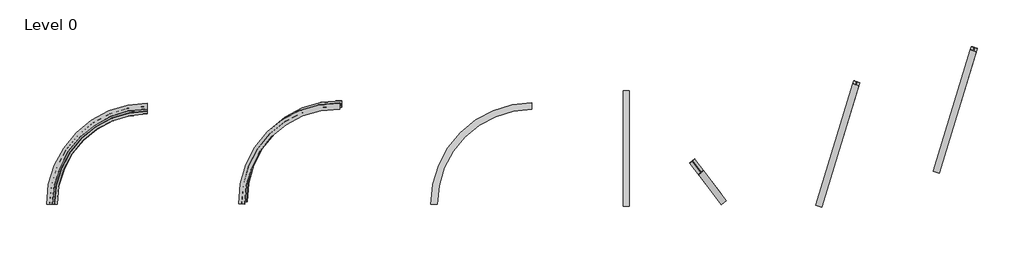
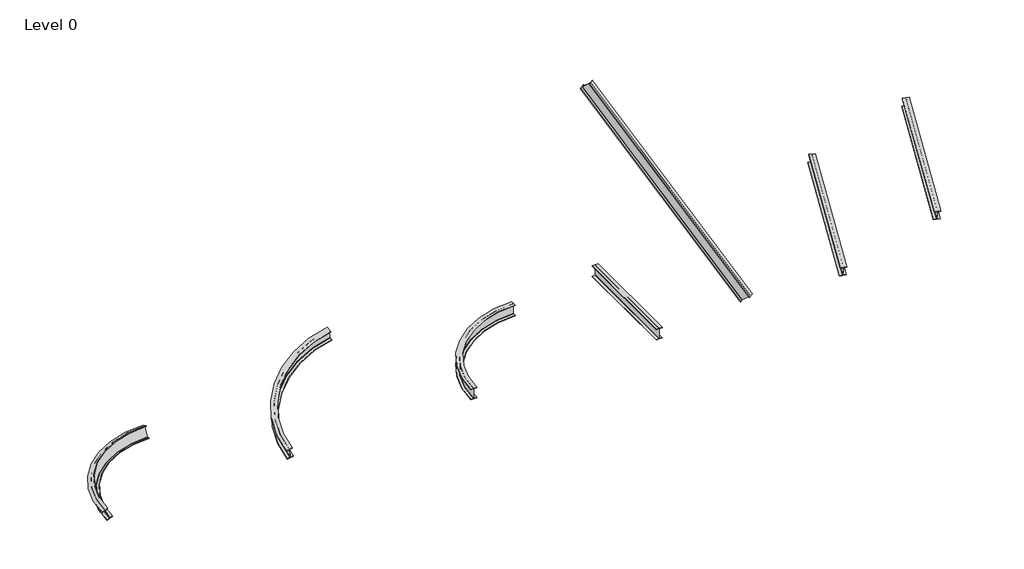
# One storey: 7 beams.
"""IFC4 building model written with IfcOpenShell, lengths in millimetres."""

import ifcopenshell
import ifcopenshell.guid

model = None  # the IFC model being written
_history = None  # IfcOwnerHistory: only IFC2X3 demands one
_inside = {}  # id of a spatial element -> (the spatial element, [elements in it])
_under = {}  # id of a project, library or spatial element -> (it, [spatial elements below it])
_declared = {}  # id of a project -> (the project, [libraries it declares])
_typed = {}  # id of a type object -> (the type object, [elements of that type])
_made_of = {}  # id of a material, layer set ... -> (it, [elements and type objects made of it])


def new_model(schema):
    """Start an empty IFC model of exactly this schema.

    Asked for "IFC4X3", IfcOpenShell would pick the latest addendum, in which some entities
    have other attributes; the version numbers below select the first issue.
    IFC2X3 requires an IfcOwnerHistory on every rooted entity: one is made here for all.
    """
    global model, _history
    if schema == "IFC4X3":
        model = ifcopenshell.file(schema_version=(4, 3, 0, 0))
    else:
        model = ifcopenshell.file(schema=schema)
    _inside.clear()
    _under.clear()
    _declared.clear()
    _typed.clear()
    _made_of.clear()
    _history = None
    if model.schema == "IFC2X3":
        org = make("IfcOrganization", Name="unknown")
        user = make(
            "IfcPersonAndOrganization",
            ThePerson=make("IfcPerson", FamilyName="unknown"),
            TheOrganization=org,
        )
        app = make(
            "IfcApplication",
            ApplicationDeveloper=org,
            Version="unknown",
            ApplicationFullName="unknown",
            ApplicationIdentifier="unknown",
        )
        _history = make(
            "IfcOwnerHistory",
            OwningUser=user,
            OwningApplication=app,
            ChangeAction="ADDED",
            CreationDate=0,
        )
    return model


def make(cls, **values):
    """One entity of the class cls with the attributes given. An attribute that is None is left unset."""
    return model.create_entity(
        cls, **{name: value for name, value in values.items() if value is not None}
    )


def rooted(cls, **values):
    """An entity with a GlobalId (a new one), such as an element, a storey or a relation."""
    return make(cls, GlobalId=ifcopenshell.guid.new(), OwnerHistory=_history, **values)


def si_unit(unit_type, name, prefix=None):
    """IfcSIUnit, for example si_unit("LENGTHUNIT", "METRE", prefix="MILLI")."""
    return make("IfcSIUnit", UnitType=unit_type, Prefix=prefix, Name=name)


def assignment(units):
    """IfcUnitAssignment: the units of a project."""
    return None if units is None else make("IfcUnitAssignment", Units=units)


def point(xyz):
    """IfcCartesianPoint."""
    return None if xyz is None else make("IfcCartesianPoint", Coordinates=xyz)


def direction(xyz):
    """IfcDirection."""
    return None if xyz is None else make("IfcDirection", DirectionRatios=xyz)


def frame(location, z_axis=None, x_axis=None):
    """IfcAxis2Placement3D, a coordinate frame: its origin and axes. An axis left out is left unset."""
    return make(
        "IfcAxis2Placement3D",
        Location=point(location),
        Axis=direction(z_axis),
        RefDirection=direction(x_axis),
    )


def frame_2d(location, x_axis=None):
    """IfcAxis2Placement2D, a coordinate frame in the plane: its origin and x axis."""
    return make(
        "IfcAxis2Placement2D", Location=point(location), RefDirection=direction(x_axis)
    )


def origin():
    """The frame at (0, 0, 0) with its axes left unset."""
    return frame((0.0, 0.0, 0.0))


def place(relative_to, where):
    """IfcLocalPlacement: puts the frame where relative to a parent placement (None: the world)."""
    return make(
        "IfcLocalPlacement", PlacementRelTo=relative_to, RelativePlacement=where
    )


def context(
    kind, dimensions, precision=None, world=None, true_north=None, identifier=None
):
    """IfcGeometricRepresentationContext, for example the 3D "Model" context."""
    return make(
        "IfcGeometricRepresentationContext",
        ContextIdentifier=identifier,
        ContextType=kind,
        CoordinateSpaceDimension=dimensions,
        Precision=precision,
        WorldCoordinateSystem=world,
        TrueNorth=true_north,
    )


def project(units=None, contexts=None):
    """IfcProject with its units and contexts."""
    return rooted(
        "IfcProject",
        Name="project",
        RepresentationContexts=contexts,
        UnitsInContext=assignment(units),
    )


def spatial(cls, under=None, at=None, **own):
    """A site, building, storey or space (cls), placed at a placement, below another one or the project."""
    s = rooted(cls, ObjectPlacement=at, **own)
    if under is not None:
        _under.setdefault(under.id(), (under, []))[1].append(s)
    return s


def polyline(points):
    """IfcPolyline through the points."""
    return make("IfcPolyline", Points=[point(p) for p in points])


def circle_curve(where, radius):
    """IfcCircle in the frame where."""
    return make("IfcCircle", Position=where, Radius=radius)


def ellipse_curve(where, semi_axis1, semi_axis2):
    """IfcEllipse in the frame where."""
    return make(
        "IfcEllipse", Position=where, SemiAxis1=semi_axis1, SemiAxis2=semi_axis2
    )


def trimmed(basis, trim1, trim2, sense, master):
    """IfcTrimmedCurve: the piece of a basis curve between two trims."""
    return make(
        "IfcTrimmedCurve",
        BasisCurve=basis,
        Trim1=trim1,
        Trim2=trim2,
        SenseAgreement=sense,
        MasterRepresentation=master,
    )


def segment(curve, same_sense, transition):
    """IfcCompositeCurveSegment."""
    return make(
        "IfcCompositeCurveSegment",
        Transition=transition,
        SameSense=same_sense,
        ParentCurve=curve,
    )


def composite_curve(segments, self_intersect=None):
    """IfcCompositeCurve: segments joined end to end."""
    return make("IfcCompositeCurve", Segments=segments, SelfIntersect=self_intersect)


def outline(outer, holes=None, kind="AREA"):
    """IfcArbitraryClosedProfileDef: a profile drawn as a closed curve; with holes, ...WithVoids."""
    if holes is None:
        return make("IfcArbitraryClosedProfileDef", ProfileType=kind, OuterCurve=outer)
    return make(
        "IfcArbitraryProfileDefWithVoids",
        ProfileType=kind,
        OuterCurve=outer,
        InnerCurves=holes,
    )


def extrude(swept, where, along, depth):
    """IfcExtrudedAreaSolid: the profile swept, set in the frame where, extruded along a direction by depth."""
    return make(
        "IfcExtrudedAreaSolid",
        SweptArea=swept,
        Position=where,
        ExtrudedDirection=direction(along),
        Depth=depth,
    )


def shape(context_of_items, identifier, shape_type, items):
    """IfcShapeRepresentation: the items that make up one representation, for example the "Body"."""
    return make(
        "IfcShapeRepresentation",
        ContextOfItems=context_of_items,
        RepresentationIdentifier=identifier,
        RepresentationType=shape_type,
        Items=items,
    )


def source(mapping_origin, context_of_items, identifier, shape_type, items):
    """IfcRepresentationMap: a shape defined once, which mapped items show again and again."""
    return make(
        "IfcRepresentationMap",
        MappingOrigin=mapping_origin,
        MappedRepresentation=shape(context_of_items, identifier, shape_type, items),
    )


def transform(
    local_origin,
    x_axis=None,
    y_axis=None,
    z_axis=None,
    scale=None,
    scale2=None,
    scale3=None,
    uniform=True,
):
    """IfcCartesianTransformationOperator3D, or its non-uniform kind. x_axis, y_axis, z_axis: its Axis1, 2, 3."""
    if uniform:
        return make(
            "IfcCartesianTransformationOperator3D",
            Axis1=direction(x_axis),
            Axis2=direction(y_axis),
            LocalOrigin=point(local_origin),
            Scale=scale,
            Axis3=direction(z_axis),
        )
    return make(
        "IfcCartesianTransformationOperator3DnonUniform",
        Axis1=direction(x_axis),
        Axis2=direction(y_axis),
        LocalOrigin=point(local_origin),
        Scale=scale,
        Axis3=direction(z_axis),
        Scale2=scale2,
        Scale3=scale3,
    )


def mapped(mapping_source, mapping_target):
    """IfcMappedItem: shows the shape of a source again, moved by a transform."""
    return make(
        "IfcMappedItem", MappingSource=mapping_source, MappingTarget=mapping_target
    )


def made_of(thing, what):
    """Note that an element or type object is made of a material, layer set ...; save() writes the relation."""
    if what is not None:
        _made_of.setdefault(what.id(), (what, []))[1].append(thing)
    return thing


def element(
    cls,
    number,
    at=None,
    inside=None,
    cuts=None,
    type_object=None,
    material=None,
    context=None,
    identifier="Body",
    shape_type=None,
    held_by="IfcProductDefinitionShape",
    body=None,
    shapes=None,
    **own,
):
    """One element of the class cls, such as IfcWall. Its Tag is "e" and its number.

    at: its placement. inside: the storey or other place that contains it. cuts: it is an
    opening in that element (IfcRelVoidsElement). A single representation is given by context,
    identifier, shape_type and body (its items); several are given by shapes. held_by: the class
    of the entity that holds the representations. save() writes the other relations.
    """
    e = rooted(cls, Tag="e%d" % number, ObjectPlacement=at, **own)
    if body is not None:
        shapes = [shape(context, identifier, shape_type, body)]
    if shapes is not None:
        e.Representation = make(held_by, Representations=shapes)
    if inside is not None:
        _inside.setdefault(inside.id(), (inside, []))[1].append(e)
    if cuts is not None:
        rooted(
            "IfcRelVoidsElement", RelatingBuildingElement=cuts, RelatedOpeningElement=e
        )
    if type_object is not None:
        _typed.setdefault(type_object.id(), (type_object, []))[1].append(e)
    return made_of(e, material)


def aggregate(whole, parts):
    """IfcRelAggregates: a whole, such as a stair, and the parts it consists of."""
    return rooted("IfcRelAggregates", RelatingObject=whole, RelatedObjects=parts)


def save(model, path):
    """Write the relations noted so far, then the file.

    IfcRelAggregates (storeys below a building ...), IfcRelContainedInSpatialStructure (elements
    in a storey), IfcRelDefinesByType, IfcRelAssociatesMaterial and IfcRelDeclares: one each for
    every whole, place, type object, material and project.
    """
    for whole, parts in _under.values():
        aggregate(whole, parts)
    for where, things in _inside.values():
        rooted(
            "IfcRelContainedInSpatialStructure",
            RelatedElements=things,
            RelatingStructure=where,
        )
    for kind, things in _typed.values():
        rooted("IfcRelDefinesByType", RelatedObjects=things, RelatingType=kind)
    for what, things in _made_of.values():
        rooted("IfcRelAssociatesMaterial", RelatedObjects=things, RelatingMaterial=what)
    for by, libraries in _declared.values():
        rooted("IfcRelDeclares", RelatingContext=by, RelatedDefinitions=libraries)
    model.write(path)


def plane_surface(at):
    """IfcPlane: the flat surface through the origin of the frame at, square to its z axis."""
    return make("IfcPlane", Position=at)


def cylinder_surface(at, radius):
    """IfcCylindricalSurface: all points at the distance radius from the z axis of the frame at."""
    return make("IfcCylindricalSurface", Position=at, Radius=radius)


def revolved_surface(curve, axis_point, axis_direction):
    """IfcSurfaceOfRevolution: the curve turned about the line through axis_point along axis_direction."""
    return make(
        "IfcSurfaceOfRevolution",
        SweptCurve=make("IfcArbitraryOpenProfileDef", ProfileType="CURVE", Curve=curve),
        AxisPosition=make("IfcAxis1Placement", Location=point(axis_point), Axis=direction(axis_direction)),
    )


def advanced_brep(points, edges, surfaces, faces):
    """IfcAdvancedBrep: a solid bounded by faces that lie on surfaces and meet in shared edges.

    An edge is (start, end): straight between two places in points (the first is 0);
    or (start, end, curve); or (start, end, curve, False) where it runs against its curve.
    A face is (place in surfaces, loops), or (place, loops, False) where it looks against
    its surface's normal. A loop lists edges by number (the first is 1), with a minus sign
    where the edge is run from its end to its start. The first loop is the outer one.
    """
    corners = [point(p) for p in points]
    vertices = [make("IfcVertexPoint", VertexGeometry=c) for c in corners]
    made = []
    for start, end, *more in edges:
        made.append(
            make(
                "IfcEdgeCurve",
                EdgeStart=vertices[start],
                EdgeEnd=vertices[end],
                EdgeGeometry=more[0] if more else make("IfcPolyline", Points=[corners[start], corners[end]]),
                SameSense=more[1] if len(more) > 1 else True,
            )
        )
    hull = []
    for where, loops, *sense in faces:
        bounds = []
        for j, loop in enumerate(loops):
            ring = [make("IfcOrientedEdge", EdgeElement=made[abs(k) - 1], Orientation=k > 0) for k in loop]
            bounds.append(
                make(
                    "IfcFaceOuterBound" if j == 0 else "IfcFaceBound",
                    Bound=make("IfcEdgeLoop", EdgeList=ring),
                    Orientation=True,
                )
            )
        hull.append(make("IfcAdvancedFace", Bounds=bounds, FaceSurface=surfaces[where], SameSense=sense[0] if sense else True))
    return make("IfcAdvancedBrep", Outer=make("IfcClosedShell", CfsFaces=hull))


def ub_universal_beams_ub305x165x40_8b2c45c1(model_context):
    return source(origin(), model_context, "Body", "SweptSolid", [
        extrude(outline(composite_curve([segment(polyline([(82.5, -141.5), (82.5, -151.7), (-82.5, -151.7), (-82.5, -141.5), (-11.9, -141.5)]), True, "CONTINUOUS"), segment(trimmed(circle_curve(frame_2d((-11.9, -132.6)), 8.9), [point((-11.9, -141.5))], [point((-3.0, -132.6))], True, "CARTESIAN"), True, "CONTINUOUS"), segment(polyline([(-3.0, -132.6), (-3.0, 132.6)]), True, "CONTINUOUS"), segment(trimmed(circle_curve(frame_2d((-11.9, 132.6)), 8.9), [point((-3.0, 132.6))], [point((-11.9, 141.5))], True, "CARTESIAN"), True, "CONTINUOUS"), segment(polyline([(-11.9, 141.5), (-82.5, 141.5), (-82.5, 151.7), (82.5, 151.7), (82.5, 141.5), (11.9, 141.5)]), True, "CONTINUOUS"), segment(trimmed(circle_curve(frame_2d((11.9, 132.6)), 8.9), [point((11.9, 141.5))], [point((3.0, 132.6))], True, "CARTESIAN"), True, "CONTINUOUS"), segment(polyline([(3.0, 132.6), (3.0, -132.6)]), True, "CONTINUOUS"), segment(trimmed(circle_curve(frame_2d((11.9, -132.6)), 8.9), [point((3.0, -132.6))], [point((11.9, -141.5))], True, "CARTESIAN"), True, "CONTINUOUS"), segment(polyline([(11.9, -141.5), (82.5, -141.5)]), True, "CONTINUOUS")], self_intersect=False)), frame((-1500.0, 0.0, 0.0), z_axis=(1.0, 0.0, 0.0), x_axis=(0.0, 1.0, 0.0)), (0.0, 0.0, 1.0), 3000.0),
    ])


def ub_universal_beams_ub305x165x40_daa15f39(model_context):
    return source(origin(), model_context, "Body", "SweptSolid", [
        extrude(outline(composite_curve([segment(polyline([(82.5, -141.5), (82.5, -151.7), (-82.5, -151.7), (-82.5, -141.5), (-11.9, -141.5)]), True, "CONTINUOUS"), segment(trimmed(circle_curve(frame_2d((-11.9, -132.6)), 8.9), [point((-11.9, -141.5))], [point((-3.0, -132.6))], True, "CARTESIAN"), True, "CONTINUOUS"), segment(polyline([(-3.0, -132.6), (-3.0, 132.6)]), True, "CONTINUOUS"), segment(trimmed(circle_curve(frame_2d((-11.9, 132.6)), 8.9), [point((-3.0, 132.6))], [point((-11.9, 141.5))], True, "CARTESIAN"), True, "CONTINUOUS"), segment(polyline([(-11.9, 141.5), (-82.5, 141.5), (-82.5, 151.7), (82.5, 151.7), (82.5, 141.5), (11.9, 141.5)]), True, "CONTINUOUS"), segment(trimmed(circle_curve(frame_2d((11.9, 132.6)), 8.9), [point((11.9, 141.5))], [point((3.0, 132.6))], True, "CARTESIAN"), True, "CONTINUOUS"), segment(polyline([(3.0, 132.6), (3.0, -132.6)]), True, "CONTINUOUS"), segment(trimmed(circle_curve(frame_2d((11.9, -132.6)), 8.9), [point((3.0, -132.6))], [point((11.9, -141.5))], True, "CARTESIAN"), True, "CONTINUOUS"), segment(polyline([(11.9, -141.5), (82.5, -141.5)]), True, "CONTINUOUS")], self_intersect=False)), frame((-1724.05, 0.0, 0.0), z_axis=(1.0, 0.0, 0.0), x_axis=(0.0, 1.0, 0.0)), (0.0, 0.0, 1.0), 3448.1),
    ])


def ub_universal_beams_ub305x165x40_ea4b1fef(model_context):
    return source(origin(), model_context, "Body", "AdvancedBrep", [
        advanced_brep(
        [(2628.0844123, -2545.5844123, -141.5), (2557.4844123, -2545.5844123, -141.5), (2548.5844123, -2545.5844123, -132.6), (2548.5844123, -2545.5844123, 132.6), (2557.4844123, -2545.5844123, 141.5), (2628.0844123, -2545.5844123, 141.5), (2628.0844123, -2545.5844123, 151.7), (2463.0844123, -2545.5844123, 151.7), (2463.0844123, -2545.5844123, 141.5), (2533.6844123, -2545.5844123, 141.5), (2542.5844123, -2545.5844123, 132.6), (2542.5844123, -2545.5844123, -132.6), (2533.6844123, -2545.5844123, -141.5), (2463.0844123, -2545.5844123, -141.5), (2463.0844123, -2545.5844123, -151.7), (2628.0844123, -2545.5844123, -151.7), (0.0, 82.5, -141.5), (0.0, 82.5, -151.7), (0.0, -82.5, -151.7), (0.0, -82.5, -141.5), (0.0, -11.9, -141.5), (0.0, -3.0, -132.6), (0.0, -3.0, 132.6), (0.0, -11.9, 141.5), (0.0, -82.5, 141.5), (0.0, -82.5, 151.7), (0.0, 82.5, 151.7), (0.0, 82.5, 141.5), (0.0, 11.9, 141.5), (0.0, 3.0, 132.6), (0.0, 3.0, -132.6), (0.0, 11.9, -141.5)],
        [
            (0, 1),
            (1, 2, circle_curve(frame((2557.4844123, -2545.5844123, -132.6), z_axis=(0.0, 1.0, 0.0), x_axis=(-1.0, 0.0, 0.0)), 8.9)),
            (2, 3),
            (3, 4, circle_curve(frame((2557.4844123, -2545.5844123, 132.6), z_axis=(0.0, 1.0, 0.0), x_axis=(-1.0, 0.0, 0.0)), 8.9)),
            (4, 5),
            (5, 6),
            (6, 7),
            (7, 8),
            (8, 9),
            (9, 10, circle_curve(frame((2533.6844123, -2545.5844123, 132.6), z_axis=(0.0, 1.0, 0.0), x_axis=(-1.0, 0.0, 0.0)), 8.9)),
            (10, 11),
            (11, 12, circle_curve(frame((2533.6844123, -2545.5844123, -132.6), z_axis=(0.0, 1.0, 0.0), x_axis=(-1.0, 0.0, 0.0)), 8.9)),
            (12, 13),
            (13, 14),
            (14, 15),
            (15, 0),
            (16, 17),
            (17, 18),
            (18, 19),
            (19, 20),
            (20, 21, circle_curve(frame((0.0, -11.9, -132.6), z_axis=(1.0, 0.0, 0.0), x_axis=(0.0, -1.0, 0.0)), 8.9)),
            (21, 22),
            (22, 23, circle_curve(frame((0.0, -11.9, 132.6), z_axis=(1.0, 0.0, 0.0), x_axis=(0.0, -1.0, 0.0)), 8.9)),
            (23, 24),
            (24, 25),
            (25, 26),
            (26, 27),
            (27, 28),
            (28, 29, circle_curve(frame((0.0, 11.9, 132.6), z_axis=(1.0, 0.0, 0.0), x_axis=(0.0, -1.0, 0.0)), 8.9)),
            (29, 30),
            (30, 31, circle_curve(frame((0.0, 11.9, -132.6), z_axis=(1.0, 0.0, 0.0), x_axis=(0.0, -1.0, 0.0)), 8.9)),
            (31, 16),
            (0, 16, circle_curve(frame((0.0, -2545.5844123, -141.5), z_axis=(0.0, 0.0, 1.0), x_axis=(0.0, 1.0, 0.0)), 2628.0844123)),
            (31, 1, circle_curve(frame((0.0, -2545.5844123, -141.5), z_axis=(0.0, 0.0, -1.0), x_axis=(0.0, 1.0, 0.0)), 2557.4844123)),
            (30, 2, circle_curve(frame((0.0, -2545.5844123, -132.6), z_axis=(0.0, 0.0, -1.0), x_axis=(0.0, 1.0, 0.0)), 2548.5844123)),
            (29, 3, circle_curve(frame((0.0, -2545.5844123, 132.6), z_axis=(0.0, 0.0, -1.0), x_axis=(0.0, 1.0, 0.0)), 2548.5844123)),
            (28, 4, circle_curve(frame((0.0, -2545.5844123, 141.5), z_axis=(0.0, 0.0, -1.0), x_axis=(0.0, 1.0, 0.0)), 2557.4844123)),
            (27, 5, circle_curve(frame((0.0, -2545.5844123, 141.5), z_axis=(0.0, 0.0, -1.0), x_axis=(0.0, 1.0, 0.0)), 2628.0844123)),
            (26, 6, circle_curve(frame((0.0, -2545.5844123, 151.7), z_axis=(0.0, 0.0, -1.0), x_axis=(0.0, 1.0, 0.0)), 2628.0844123)),
            (25, 7, circle_curve(frame((0.0, -2545.5844123, 151.7), z_axis=(0.0, 0.0, -1.0), x_axis=(0.0, 1.0, 0.0)), 2463.0844123)),
            (24, 8, circle_curve(frame((0.0, -2545.5844123, 141.5), z_axis=(0.0, 0.0, -1.0), x_axis=(0.0, 1.0, 0.0)), 2463.0844123)),
            (23, 9, circle_curve(frame((0.0, -2545.5844123, 141.5), z_axis=(0.0, 0.0, -1.0), x_axis=(0.0, 1.0, 0.0)), 2533.6844123)),
            (22, 10, circle_curve(frame((0.0, -2545.5844123, 132.6), z_axis=(0.0, 0.0, -1.0), x_axis=(0.0, 1.0, 0.0)), 2542.5844123)),
            (21, 11, circle_curve(frame((0.0, -2545.5844123, -132.6), z_axis=(0.0, 0.0, -1.0), x_axis=(0.0, 1.0, 0.0)), 2542.5844123)),
            (20, 12, circle_curve(frame((0.0, -2545.5844123, -141.5), z_axis=(0.0, 0.0, -1.0), x_axis=(0.0, 1.0, 0.0)), 2533.6844123)),
            (19, 13, circle_curve(frame((0.0, -2545.5844123, -141.5), z_axis=(0.0, 0.0, -1.0), x_axis=(0.0, 1.0, 0.0)), 2463.0844123)),
            (18, 14, circle_curve(frame((0.0, -2545.5844123, -151.7), z_axis=(0.0, 0.0, -1.0), x_axis=(0.0, 1.0, 0.0)), 2463.0844123)),
            (17, 15, circle_curve(frame((0.0, -2545.5844123, -151.7), z_axis=(0.0, 0.0, -1.0), x_axis=(0.0, 1.0, 0.0)), 2628.0844123)),
        ],
        [
            plane_surface(frame((2545.5844123, -2545.5844123, 0.0), z_axis=(0.0, -1.0, 0.0), x_axis=(0.0, 0.0, 1.0))),
            plane_surface(frame((0.0, 0.0, 0.0), z_axis=(-1.0, 0.0, 0.0), x_axis=(0.0, 0.0, 1.0))),
            plane_surface(frame((0.0, -2545.5844123, -141.5), z_axis=(0.0, 0.0, 1.0), x_axis=(0.0, 1.0, 0.0))),
            revolved_surface(trimmed(ellipse_curve(frame((0.0, 11.9, -132.6), z_axis=(1.0, 0.0, 0.0), x_axis=(0.0, -1.0, 0.0)), 8.9, 8.9), [point((0.0, 3.0, -132.6))], [point((0.0, 11.9, -141.5))], True, "CARTESIAN"), (0.0, -2545.5844123, 0.0), (0.0, 0.0, -1.0)),
            cylinder_surface(frame((0.0, -2545.5844123, 0.0), z_axis=(0.0, 0.0, -1.0), x_axis=(0.0, 1.0, 0.0)), 2548.5844123),
            revolved_surface(trimmed(ellipse_curve(frame((0.0, 11.9, 132.6), z_axis=(1.0, 0.0, 0.0), x_axis=(0.0, -1.0, 0.0)), 8.9, 8.9), [point((0.0, 11.9, 141.5))], [point((0.0, 3.0, 132.6))], True, "CARTESIAN"), (0.0, -2545.5844123, 0.0), (0.0, 0.0, -1.0)),
            plane_surface(frame((0.0, -2545.5844123, 141.5), z_axis=(0.0, 0.0, -1.0), x_axis=(0.0, 1.0, 0.0))),
            cylinder_surface(frame((0.0, -2545.5844123, 0.0), z_axis=(0.0, 0.0, -1.0), x_axis=(0.0, 1.0, 0.0)), 2628.0844123),
            plane_surface(frame((0.0, -2545.5844123, 151.7), z_axis=(0.0, 0.0, 1.0), x_axis=(0.0, 1.0, 0.0))),
            revolved_surface(polyline([(0.0, -82.5, 141.5), (0.0, -82.5, 151.7)]), (0.0, -2545.5844123, 0.0), (0.0, 0.0, -1.0)),
            revolved_surface(trimmed(ellipse_curve(frame((0.0, -11.9, 132.6), z_axis=(1.0, 0.0, 0.0), x_axis=(0.0, -1.0, 0.0)), 8.9, 8.9), [point((0.0, -3.0, 132.6))], [point((0.0, -11.9, 141.5))], True, "CARTESIAN"), (0.0, -2545.5844123, 0.0), (0.0, 0.0, -1.0)),
            revolved_surface(polyline([(0.0, -3.0, -132.6), (0.0, -3.0, 132.6)]), (0.0, -2545.5844123, 0.0), (0.0, 0.0, -1.0)),
            revolved_surface(trimmed(ellipse_curve(frame((0.0, -11.9, -132.6), z_axis=(1.0, 0.0, 0.0), x_axis=(0.0, -1.0, 0.0)), 8.9, 8.9), [point((0.0, -11.9, -141.5))], [point((0.0, -3.0, -132.6))], True, "CARTESIAN"), (0.0, -2545.5844123, 0.0), (0.0, 0.0, -1.0)),
            revolved_surface(polyline([(0.0, -82.5, -151.7), (0.0, -82.5, -141.5)]), (0.0, -2545.5844123, 0.0), (0.0, 0.0, -1.0)),
            plane_surface(frame((0.0, -2545.5844123, -151.7), z_axis=(0.0, 0.0, -1.0), x_axis=(0.0, 1.0, 0.0))),
        ],
        [
            (0, [[1, 2, 3, 4, 5, 6, 7, 8, 9, 10, 11, 12, 13, 14, 15, 16]]),
            (1, [[17, 18, 19, 20, 21, 22, 23, 24, 25, 26, 27, 28, 29, 30, 31, 32]]),
            (2, [[-1, 33, -32, 34]]),
            (3, [[-2, -34, -31, 35]]),
            (4, [[-3, -35, -30, 36]]),
            (5, [[-4, -36, -29, 37]]),
            (6, [[-5, -37, -28, 38]]),
            (7, [[-6, -38, -27, 39]]),
            (8, [[-7, -39, -26, 40]]),
            (9, [[-8, -40, -25, 41]]),
            (6, [[-9, -41, -24, 42]]),
            (10, [[-10, -42, -23, 43]]),
            (11, [[-11, -43, -22, 44]]),
            (12, [[-12, -44, -21, 45]]),
            (2, [[-13, -45, -20, 46]]),
            (13, [[-14, -46, -19, 47]]),
            (14, [[-15, -47, -18, 48]]),
            (7, [[-16, -48, -17, -33]]),
        ],
    ),
    ])


def ub_universal_beams_ub305x165x40_a7bc032b(model_context):
    return source(origin(), model_context, "Body", "AdvancedBrep", [
        advanced_brep(
        [(2724.4689627, -2641.9689627, -141.5), (2653.8689627, -2641.9689627, -141.5), (2644.9689627, -2641.9689627, -132.6), (2644.9689627, -2641.9689627, 132.6), (2653.8689627, -2641.9689627, 141.5), (2724.4689627, -2641.9689627, 141.5), (2724.4689627, -2641.9689627, 151.7), (2559.4689627, -2641.9689627, 151.7), (2559.4689627, -2641.9689627, 141.5), (2630.0689627, -2641.9689627, 141.5), (2638.9689627, -2641.9689627, 132.6), (2638.9689627, -2641.9689627, -132.6), (2630.0689627, -2641.9689627, -141.5), (2559.4689627, -2641.9689627, -141.5), (2559.4689627, -2641.9689627, -151.7), (2724.4689627, -2641.9689627, -151.7), (0.0, 82.5, -141.5), (0.0, 82.5, -151.7), (0.0, -82.5, -151.7), (0.0, -82.5, -141.5), (0.0, -11.9, -141.5), (0.0, -3.0, -132.6), (0.0, -3.0, 132.6), (0.0, -11.9, 141.5), (0.0, -82.5, 141.5), (0.0, -82.5, 151.7), (0.0, 82.5, 151.7), (0.0, 82.5, 141.5), (0.0, 11.9, 141.5), (0.0, 3.0, 132.6), (0.0, 3.0, -132.6), (0.0, 11.9, -141.5)],
        [
            (0, 1),
            (1, 2, circle_curve(frame((2653.8689627, -2641.9689627, -132.6), z_axis=(0.0, 1.0, 0.0), x_axis=(-1.0, 0.0, 0.0)), 8.9)),
            (2, 3),
            (3, 4, circle_curve(frame((2653.8689627, -2641.9689627, 132.6), z_axis=(0.0, 1.0, 0.0), x_axis=(-1.0, 0.0, 0.0)), 8.9)),
            (4, 5),
            (5, 6),
            (6, 7),
            (7, 8),
            (8, 9),
            (9, 10, circle_curve(frame((2630.0689627, -2641.9689627, 132.6), z_axis=(0.0, 1.0, 0.0), x_axis=(-1.0, 0.0, 0.0)), 8.9)),
            (10, 11),
            (11, 12, circle_curve(frame((2630.0689627, -2641.9689627, -132.6), z_axis=(0.0, 1.0, 0.0), x_axis=(-1.0, 0.0, 0.0)), 8.9)),
            (12, 13),
            (13, 14),
            (14, 15),
            (15, 0),
            (16, 17),
            (17, 18),
            (18, 19),
            (19, 20),
            (20, 21, circle_curve(frame((0.0, -11.9, -132.6), z_axis=(1.0, 0.0, 0.0), x_axis=(0.0, -1.0, 0.0)), 8.9)),
            (21, 22),
            (22, 23, circle_curve(frame((0.0, -11.9, 132.6), z_axis=(1.0, 0.0, 0.0), x_axis=(0.0, -1.0, 0.0)), 8.9)),
            (23, 24),
            (24, 25),
            (25, 26),
            (26, 27),
            (27, 28),
            (28, 29, circle_curve(frame((0.0, 11.9, 132.6), z_axis=(1.0, 0.0, 0.0), x_axis=(0.0, -1.0, 0.0)), 8.9)),
            (29, 30),
            (30, 31, circle_curve(frame((0.0, 11.9, -132.6), z_axis=(1.0, 0.0, 0.0), x_axis=(0.0, -1.0, 0.0)), 8.9)),
            (31, 16),
            (0, 16, circle_curve(frame((0.0, -2641.9689627, -141.5), z_axis=(0.0, 0.0, 1.0), x_axis=(0.0, 1.0, 0.0)), 2724.4689627)),
            (31, 1, circle_curve(frame((0.0, -2641.9689627, -141.5), z_axis=(0.0, 0.0, -1.0), x_axis=(0.0, 1.0, 0.0)), 2653.8689627)),
            (30, 2, circle_curve(frame((0.0, -2641.9689627, -132.6), z_axis=(0.0, 0.0, -1.0), x_axis=(0.0, 1.0, 0.0)), 2644.9689627)),
            (29, 3, circle_curve(frame((0.0, -2641.9689627, 132.6), z_axis=(0.0, 0.0, -1.0), x_axis=(0.0, 1.0, 0.0)), 2644.9689627)),
            (28, 4, circle_curve(frame((0.0, -2641.9689627, 141.5), z_axis=(0.0, 0.0, -1.0), x_axis=(0.0, 1.0, 0.0)), 2653.8689627)),
            (27, 5, circle_curve(frame((0.0, -2641.9689627, 141.5), z_axis=(0.0, 0.0, -1.0), x_axis=(0.0, 1.0, 0.0)), 2724.4689627)),
            (26, 6, circle_curve(frame((0.0, -2641.9689627, 151.7), z_axis=(0.0, 0.0, -1.0), x_axis=(0.0, 1.0, 0.0)), 2724.4689627)),
            (25, 7, circle_curve(frame((0.0, -2641.9689627, 151.7), z_axis=(0.0, 0.0, -1.0), x_axis=(0.0, 1.0, 0.0)), 2559.4689627)),
            (24, 8, circle_curve(frame((0.0, -2641.9689627, 141.5), z_axis=(0.0, 0.0, -1.0), x_axis=(0.0, 1.0, 0.0)), 2559.4689627)),
            (23, 9, circle_curve(frame((0.0, -2641.9689627, 141.5), z_axis=(0.0, 0.0, -1.0), x_axis=(0.0, 1.0, 0.0)), 2630.0689627)),
            (22, 10, circle_curve(frame((0.0, -2641.9689627, 132.6), z_axis=(0.0, 0.0, -1.0), x_axis=(0.0, 1.0, 0.0)), 2638.9689627)),
            (21, 11, circle_curve(frame((0.0, -2641.9689627, -132.6), z_axis=(0.0, 0.0, -1.0), x_axis=(0.0, 1.0, 0.0)), 2638.9689627)),
            (20, 12, circle_curve(frame((0.0, -2641.9689627, -141.5), z_axis=(0.0, 0.0, -1.0), x_axis=(0.0, 1.0, 0.0)), 2630.0689627)),
            (19, 13, circle_curve(frame((0.0, -2641.9689627, -141.5), z_axis=(0.0, 0.0, -1.0), x_axis=(0.0, 1.0, 0.0)), 2559.4689627)),
            (18, 14, circle_curve(frame((0.0, -2641.9689627, -151.7), z_axis=(0.0, 0.0, -1.0), x_axis=(0.0, 1.0, 0.0)), 2559.4689627)),
            (17, 15, circle_curve(frame((0.0, -2641.9689627, -151.7), z_axis=(0.0, 0.0, -1.0), x_axis=(0.0, 1.0, 0.0)), 2724.4689627)),
        ],
        [
            plane_surface(frame((2641.9689627, -2641.9689627, 0.0), z_axis=(0.0, -1.0, 0.0), x_axis=(0.0, 0.0, 1.0))),
            plane_surface(frame((0.0, 0.0, 0.0), z_axis=(-1.0, 0.0, 0.0), x_axis=(0.0, 0.0, 1.0))),
            plane_surface(frame((0.0, -2641.9689627, -141.5), z_axis=(0.0, 0.0, 1.0), x_axis=(0.0, 1.0, 0.0))),
            revolved_surface(trimmed(ellipse_curve(frame((0.0, 11.9, -132.6), z_axis=(1.0, 0.0, 0.0), x_axis=(0.0, -1.0, 0.0)), 8.9, 8.9), [point((0.0, 3.0, -132.6))], [point((0.0, 11.9, -141.5))], True, "CARTESIAN"), (0.0, -2641.9689627, 0.0), (0.0, 0.0, -1.0)),
            cylinder_surface(frame((0.0, -2641.9689627, 0.0), z_axis=(0.0, 0.0, -1.0), x_axis=(0.0, 1.0, 0.0)), 2644.9689627),
            revolved_surface(trimmed(ellipse_curve(frame((0.0, 11.9, 132.6), z_axis=(1.0, 0.0, 0.0), x_axis=(0.0, -1.0, 0.0)), 8.9, 8.9), [point((0.0, 11.9, 141.5))], [point((0.0, 3.0, 132.6))], True, "CARTESIAN"), (0.0, -2641.9689627, 0.0), (0.0, 0.0, -1.0)),
            plane_surface(frame((0.0, -2641.9689627, 141.5), z_axis=(0.0, 0.0, -1.0), x_axis=(0.0, 1.0, 0.0))),
            cylinder_surface(frame((0.0, -2641.9689627, 0.0), z_axis=(0.0, 0.0, -1.0), x_axis=(0.0, 1.0, 0.0)), 2724.4689627),
            plane_surface(frame((0.0, -2641.9689627, 151.7), z_axis=(0.0, 0.0, 1.0), x_axis=(0.0, 1.0, 0.0))),
            revolved_surface(polyline([(0.0, -82.5, 141.5), (0.0, -82.5, 151.7)]), (0.0, -2641.9689627, 0.0), (0.0, 0.0, -1.0)),
            revolved_surface(trimmed(ellipse_curve(frame((0.0, -11.9, 132.6), z_axis=(1.0, 0.0, 0.0), x_axis=(0.0, -1.0, 0.0)), 8.9, 8.9), [point((0.0, -3.0, 132.6))], [point((0.0, -11.9, 141.5))], True, "CARTESIAN"), (0.0, -2641.9689627, 0.0), (0.0, 0.0, -1.0)),
            revolved_surface(polyline([(0.0, -3.0, -132.6), (0.0, -3.0, 132.6)]), (0.0, -2641.9689627, 0.0), (0.0, 0.0, -1.0)),
            revolved_surface(trimmed(ellipse_curve(frame((0.0, -11.9, -132.6), z_axis=(1.0, 0.0, 0.0), x_axis=(0.0, -1.0, 0.0)), 8.9, 8.9), [point((0.0, -11.9, -141.5))], [point((0.0, -3.0, -132.6))], True, "CARTESIAN"), (0.0, -2641.9689627, 0.0), (0.0, 0.0, -1.0)),
            revolved_surface(polyline([(0.0, -82.5, -151.7), (0.0, -82.5, -141.5)]), (0.0, -2641.9689627, 0.0), (0.0, 0.0, -1.0)),
            plane_surface(frame((0.0, -2641.9689627, -151.7), z_axis=(0.0, 0.0, -1.0), x_axis=(0.0, 1.0, 0.0))),
        ],
        [
            (0, [[1, 2, 3, 4, 5, 6, 7, 8, 9, 10, 11, 12, 13, 14, 15, 16]]),
            (1, [[17, 18, 19, 20, 21, 22, 23, 24, 25, 26, 27, 28, 29, 30, 31, 32]]),
            (2, [[-1, 33, -32, 34]]),
            (3, [[-2, -34, -31, 35]]),
            (4, [[-3, -35, -30, 36]]),
            (5, [[-4, -36, -29, 37]]),
            (6, [[-5, -37, -28, 38]]),
            (7, [[-6, -38, -27, 39]]),
            (8, [[-7, -39, -26, 40]]),
            (9, [[-8, -40, -25, 41]]),
            (6, [[-9, -41, -24, 42]]),
            (10, [[-10, -42, -23, 43]]),
            (11, [[-11, -43, -22, 44]]),
            (12, [[-12, -44, -21, 45]]),
            (2, [[-13, -45, -20, 46]]),
            (13, [[-14, -46, -19, 47]]),
            (14, [[-15, -47, -18, 48]]),
            (7, [[-16, -48, -17, -33]]),
        ],
    ),
    ])


def ub_universal_beams_ub305x165x40_80cf76f0(model_context):
    return source(origin(), model_context, "Body", "AdvancedBrep", [
        advanced_brep(
        [(2496.4431304, -2481.473222, -163.1085585), (2432.4578006, -2481.473222, -133.2717092), (2428.1529638, -2481.473222, -121.4442673), (2540.2313268, -2481.473222, 118.9085578), (2552.0587687, -2481.473222, 123.2133946), (2616.0440984, -2481.473222, 93.3765453), (2620.3548047, -2481.473222, 102.6208847), (2470.8140198, -2481.473222, 172.3528979), (2466.5033136, -2481.473222, 163.1085585), (2530.4886433, -2481.473222, 133.2717092), (2534.7934801, -2481.473222, 121.4442673), (2422.7151171, -2481.473222, -118.9085578), (2410.8876753, -2481.473222, -123.2133946), (2346.9023455, -2481.473222, -93.3765453), (2342.5916392, -2481.473222, -102.6208847), (2492.1324241, -2481.473222, -172.3528979), (0.0, 14.9699084, -163.1085585), (0.0, 10.6592021, -172.3528979), (0.0, -138.8815827, -102.6208847), (0.0, -134.5708765, -93.3765453), (0.0, -70.5855467, -123.2133946), (0.0, -58.7581049, -118.9085578), (0.0, 53.3202581, 121.4442673), (0.0, 49.0154214, 133.2717092), (0.0, -14.9699084, 163.1085585), (0.0, -10.6592021, 172.3528979), (0.0, 138.8815827, 102.6208847), (0.0, 134.5708765, 93.3765453), (0.0, 70.5855467, 123.2133946), (0.0, 58.7581049, 118.9085578), (0.0, -53.3202581, -121.4442673), (0.0, -49.0154214, -133.2717092)],
        [
            (0, 1),
            (1, 2, circle_curve(frame((2436.2191031, -2481.473222, -125.2055699), z_axis=(0.0, 1.0, 0.0), x_axis=(-0.9063077870366502, 0.0, 0.4226182617406989)), 8.9)),
            (2, 3),
            (3, 4, circle_curve(frame((2548.2974661, -2481.473222, 115.1472552), z_axis=(0.0, 1.0, 0.0), x_axis=(-0.9063077870366502, 0.0, 0.4226182617406989)), 8.9)),
            (4, 5),
            (5, 6),
            (6, 7),
            (7, 8),
            (8, 9),
            (9, 10, circle_curve(frame((2526.7273408, -2481.473222, 125.2055699), z_axis=(0.0, 1.0, 0.0), x_axis=(-0.9063077870366502, 0.0, 0.4226182617406989)), 8.9)),
            (10, 11),
            (11, 12, circle_curve(frame((2414.6489778, -2481.473222, -115.1472552), z_axis=(0.0, 1.0, 0.0), x_axis=(-0.9063077870366502, 0.0, 0.4226182617406989)), 8.9)),
            (12, 13),
            (13, 14),
            (14, 15),
            (15, 0),
            (16, 17),
            (17, 18),
            (18, 19),
            (19, 20),
            (20, 21, circle_curve(frame((0.0, -66.8242442, -115.1472552), z_axis=(1.0, 0.0, 0.0), x_axis=(0.0, -0.9063077870366502, 0.422618261740699)), 8.9)),
            (21, 22),
            (22, 23, circle_curve(frame((0.0, 45.2541188, 125.2055699), z_axis=(1.0, 0.0, 0.0), x_axis=(0.0, -0.9063077870366502, 0.422618261740699)), 8.9)),
            (23, 24),
            (24, 25),
            (25, 26),
            (26, 27),
            (27, 28),
            (28, 29, circle_curve(frame((0.0, 66.8242442, 115.1472552), z_axis=(1.0, 0.0, 0.0), x_axis=(0.0, -0.9063077870366502, 0.422618261740699)), 8.9)),
            (29, 30),
            (30, 31, circle_curve(frame((0.0, -45.2541188, -125.2055699), z_axis=(1.0, 0.0, 0.0), x_axis=(0.0, -0.9063077870366502, 0.422618261740699)), 8.9)),
            (31, 16),
            (0, 16, circle_curve(frame((0.0, -2481.473222, -163.1085585), z_axis=(0.0, 0.0, 1.0), x_axis=(0.0, 1.0, 0.0)), 2496.4431304)),
            (31, 1, circle_curve(frame((0.0, -2481.473222, -133.2717092), z_axis=(0.0, 0.0, -1.0), x_axis=(0.0, 1.0, 0.0)), 2432.4578006)),
            (30, 2, circle_curve(frame((0.0, -2481.473222, -121.4442673), z_axis=(0.0, 0.0, -1.0), x_axis=(0.0, 1.0, 0.0)), 2428.1529638)),
            (29, 3, circle_curve(frame((0.0, -2481.473222, 118.9085578), z_axis=(0.0, 0.0, -1.0), x_axis=(0.0, 1.0, 0.0)), 2540.2313268)),
            (28, 4, circle_curve(frame((0.0, -2481.473222, 123.2133946), z_axis=(0.0, 0.0, -1.0), x_axis=(0.0, 1.0, 0.0)), 2552.0587687)),
            (27, 5, circle_curve(frame((0.0, -2481.473222, 93.3765453), z_axis=(0.0, 0.0, -1.0), x_axis=(0.0, 1.0, 0.0)), 2616.0440984)),
            (26, 6, circle_curve(frame((0.0, -2481.473222, 102.6208847), z_axis=(0.0, 0.0, -1.0), x_axis=(0.0, 1.0, 0.0)), 2620.3548047)),
            (25, 7, circle_curve(frame((0.0, -2481.473222, 172.3528979), z_axis=(0.0, 0.0, -1.0), x_axis=(0.0, 1.0, 0.0)), 2470.8140198)),
            (24, 8, circle_curve(frame((0.0, -2481.473222, 163.1085585), z_axis=(0.0, 0.0, -1.0), x_axis=(0.0, 1.0, 0.0)), 2466.5033136)),
            (23, 9, circle_curve(frame((0.0, -2481.473222, 133.2717092), z_axis=(0.0, 0.0, -1.0), x_axis=(0.0, 1.0, 0.0)), 2530.4886433)),
            (22, 10, circle_curve(frame((0.0, -2481.473222, 121.4442673), z_axis=(0.0, 0.0, -1.0), x_axis=(0.0, 1.0, 0.0)), 2534.7934801)),
            (21, 11, circle_curve(frame((0.0, -2481.473222, -118.9085578), z_axis=(0.0, 0.0, -1.0), x_axis=(0.0, 1.0, 0.0)), 2422.7151171)),
            (20, 12, circle_curve(frame((0.0, -2481.473222, -123.2133946), z_axis=(0.0, 0.0, -1.0), x_axis=(0.0, 1.0, 0.0)), 2410.8876753)),
            (19, 13, circle_curve(frame((0.0, -2481.473222, -93.3765453), z_axis=(0.0, 0.0, -1.0), x_axis=(0.0, 1.0, 0.0)), 2346.9023455)),
            (18, 14, circle_curve(frame((0.0, -2481.473222, -102.6208847), z_axis=(0.0, 0.0, -1.0), x_axis=(0.0, 1.0, 0.0)), 2342.5916392)),
            (17, 15, circle_curve(frame((0.0, -2481.473222, -172.3528979), z_axis=(0.0, 0.0, -1.0), x_axis=(0.0, 1.0, 0.0)), 2492.1324241)),
        ],
        [
            plane_surface(frame((2481.473222, -2481.473222, 0.0), z_axis=(0.0, -1.0, 0.0), x_axis=(0.42261826174069883, 0.0, 0.9063077870366503))),
            plane_surface(frame((0.0, 0.0, 0.0), z_axis=(-1.0, 0.0, 0.0), x_axis=(0.0, 0.422618261740699, 0.9063077870366502))),
            revolved_surface(polyline([(0.0, -49.0154214, -133.2717092), (0.0, 14.9699084, -163.1085585)]), (0.0, -2481.473222, 0.0), (0.0, 0.0, -1.0)),
            revolved_surface(trimmed(ellipse_curve(frame((0.0, -45.2541188, -125.2055699), z_axis=(1.0, 0.0, 0.0), x_axis=(0.0, -0.9063077870366502, 0.422618261740699)), 8.9, 8.9), [point((0.0, -53.3202581, -121.4442673))], [point((0.0, -49.0154214, -133.2717092))], True, "CARTESIAN"), (0.0, -2481.473222, 0.0), (0.0, 0.0, -1.0)),
            revolved_surface(polyline([(0.0, 58.7581049, 118.9085578), (0.0, -53.3202581, -121.4442673)]), (0.0, -2481.473222, 0.0), (0.0, 0.0, -1.0)),
            revolved_surface(trimmed(ellipse_curve(frame((0.0, 66.8242442, 115.1472552), z_axis=(1.0, 0.0, 0.0), x_axis=(0.0, -0.9063077870366502, 0.422618261740699)), 8.9, 8.9), [point((0.0, 70.5855467, 123.2133946))], [point((0.0, 58.7581049, 118.9085578))], True, "CARTESIAN"), (0.0, -2481.473222, 0.0), (0.0, 0.0, -1.0)),
            revolved_surface(polyline([(0.0, 134.5708765, 93.3765453), (0.0, 70.5855467, 123.2133946)]), (0.0, -2481.473222, 0.0), (0.0, 0.0, -1.0)),
            revolved_surface(polyline([(0.0, 138.8815827, 102.6208847), (0.0, 134.5708765, 93.3765453)]), (0.0, -2481.473222, 0.0), (0.0, 0.0, -1.0)),
            revolved_surface(polyline([(0.0, -10.6592021, 172.3528979), (0.0, 138.8815827, 102.6208847)]), (0.0, -2481.473222, 0.0), (0.0, 0.0, -1.0)),
            revolved_surface(polyline([(0.0, -14.9699084, 163.1085585), (0.0, -10.6592021, 172.3528979)]), (0.0, -2481.473222, 0.0), (0.0, 0.0, -1.0)),
            revolved_surface(polyline([(0.0, 49.0154214, 133.2717092), (0.0, -14.9699084, 163.1085585)]), (0.0, -2481.473222, 0.0), (0.0, 0.0, -1.0)),
            revolved_surface(trimmed(ellipse_curve(frame((0.0, 45.2541188, 125.2055699), z_axis=(1.0, 0.0, 0.0), x_axis=(0.0, -0.9063077870366502, 0.422618261740699)), 8.9, 8.9), [point((0.0, 53.3202581, 121.4442673))], [point((0.0, 49.0154214, 133.2717092))], True, "CARTESIAN"), (0.0, -2481.473222, 0.0), (0.0, 0.0, -1.0)),
            revolved_surface(polyline([(0.0, -58.7581049, -118.9085578), (0.0, 53.3202581, 121.4442673)]), (0.0, -2481.473222, 0.0), (0.0, 0.0, -1.0)),
            revolved_surface(trimmed(ellipse_curve(frame((0.0, -66.8242442, -115.1472552), z_axis=(1.0, 0.0, 0.0), x_axis=(0.0, -0.9063077870366502, 0.422618261740699)), 8.9, 8.9), [point((0.0, -70.5855467, -123.2133946))], [point((0.0, -58.7581049, -118.9085578))], True, "CARTESIAN"), (0.0, -2481.473222, 0.0), (0.0, 0.0, -1.0)),
            revolved_surface(polyline([(0.0, -134.5708765, -93.3765453), (0.0, -70.5855467, -123.2133946)]), (0.0, -2481.473222, 0.0), (0.0, 0.0, -1.0)),
            revolved_surface(polyline([(0.0, -138.8815827, -102.6208847), (0.0, -134.5708765, -93.3765453)]), (0.0, -2481.473222, 0.0), (0.0, 0.0, -1.0)),
            revolved_surface(polyline([(0.0, 10.6592021, -172.3528979), (0.0, -138.8815827, -102.6208847)]), (0.0, -2481.473222, 0.0), (0.0, 0.0, -1.0)),
            revolved_surface(polyline([(0.0, 14.9699084, -163.1085585), (0.0, 10.6592021, -172.3528979)]), (0.0, -2481.473222, 0.0), (0.0, 0.0, -1.0)),
        ],
        [
            (0, [[1, 2, 3, 4, 5, 6, 7, 8, 9, 10, 11, 12, 13, 14, 15, 16]]),
            (1, [[17, 18, 19, 20, 21, 22, 23, 24, 25, 26, 27, 28, 29, 30, 31, 32]]),
            (2, [[-1, 33, -32, 34]]),
            (3, [[-2, -34, -31, 35]]),
            (4, [[-3, -35, -30, 36]]),
            (5, [[-4, -36, -29, 37]]),
            (6, [[-5, -37, -28, 38]]),
            (7, [[-6, -38, -27, 39]]),
            (8, [[-7, -39, -26, 40]]),
            (9, [[-8, -40, -25, 41]]),
            (10, [[-9, -41, -24, 42]]),
            (11, [[-10, -42, -23, 43]]),
            (12, [[-11, -43, -22, 44]]),
            (13, [[-12, -44, -21, 45]]),
            (14, [[-13, -45, -20, 46]]),
            (15, [[-14, -46, -19, 47]]),
            (16, [[-15, -47, -18, 48]]),
            (17, [[-16, -48, -17, -33]]),
        ],
    ),
    ])


def ub_universal_beams_ub305x165x40_614cc3fe(model_context):
    return source(origin(), model_context, "Body", "SweptSolid", [
        extrude(outline(composite_curve([segment(polyline([(82.5, -141.5), (82.5, -151.7), (-82.5, -151.7), (-82.5, -141.5), (-11.9, -141.5)]), True, "CONTINUOUS"), segment(trimmed(circle_curve(frame_2d((-11.9, -132.6)), 8.9), [point((-11.9, -141.5))], [point((-3.0, -132.6))], True, "CARTESIAN"), True, "CONTINUOUS"), segment(polyline([(-3.0, -132.6), (-3.0, 132.6)]), True, "CONTINUOUS"), segment(trimmed(circle_curve(frame_2d((-11.9, 132.6)), 8.9), [point((-3.0, 132.6))], [point((-11.9, 141.5))], True, "CARTESIAN"), True, "CONTINUOUS"), segment(polyline([(-11.9, 141.5), (-82.5, 141.5), (-82.5, 151.7), (82.5, 151.7), (82.5, 141.5), (11.9, 141.5)]), True, "CONTINUOUS"), segment(trimmed(circle_curve(frame_2d((11.9, 132.6)), 8.9), [point((11.9, 141.5))], [point((3.0, 132.6))], True, "CARTESIAN"), True, "CONTINUOUS"), segment(polyline([(3.0, 132.6), (3.0, -132.6)]), True, "CONTINUOUS"), segment(trimmed(circle_curve(frame_2d((11.9, -132.6)), 8.9), [point((3.0, -132.6))], [point((11.9, -141.5))], True, "CARTESIAN"), True, "CONTINUOUS"), segment(polyline([(11.9, -141.5), (82.5, -141.5)]), True, "CONTINUOUS")], self_intersect=False)), frame((-3226.45, 0.0, 0.0), z_axis=(1.0, 0.0, 0.0), x_axis=(0.0, 1.0, 0.0)), (0.0, 0.0, 1.0), 6452.9),
    ])


model = new_model("IFC4")

# Units and contexts
model_context = context("Model", 3, world=origin())
ifc_project = project(units=[si_unit("LENGTHUNIT", "METRE", prefix="MILLI")], contexts=[model_context])

# Site, building, storey
site = spatial("IfcSite", under=ifc_project)
building = spatial("IfcBuilding", under=site)
storey = spatial("IfcBuildingStorey", under=building, Name="Level 0", Elevation=0.0)

# Beams
placement = place(None, origin())
ub_universal_beams_ub305x165x40_shape = ub_universal_beams_ub305x165x40_8b2c45c1(model_context)
element("IfcBeam", 1, ObjectType="UB-Universal Beams : UB305x165x40", at=placement, inside=storey, context=model_context, shape_type="MappedRepresentation", body=[
    mapped(ub_universal_beams_ub305x165x40_shape, transform((-15000.0, 5000.0, -151.7), x_axis=(0.0, 1.0, 0.0), y_axis=(-1.0, 0.0, 0.0), z_axis=(0.0, 0.0, 1.0))),
])
ub_universal_beams_ub305x165x40_2_shape = ub_universal_beams_ub305x165x40_daa15f39(model_context)
element("IfcBeam", 2, ObjectType="UB-Universal Beams : UB305x165x40", at=placement, inside=storey, context=model_context, shape_type="MappedRepresentation", body=[
    mapped(ub_universal_beams_ub305x165x40_2_shape, transform((-9504.7240508, 5119.9746353, 354.8193978), x_axis=(0.27980685658547805, 0.9152069895324219, 0.2900073952828708), y_axis=(-0.9563047559630351, 0.2923717047227384, 0.0), z_axis=(-0.08478995654105395, -0.27733545137346116, 0.9570244044334736))),
])
element("IfcBeam", 3, ObjectType="UB-Universal Beams : UB305x165x40", at=placement, inside=storey, context=model_context, shape_type="MappedRepresentation", body=[
    mapped(ub_universal_beams_ub305x165x40_2_shape, transform((-6444.0004096, 6006.8128035, 354.8193978), x_axis=(0.27980685658547805, 0.9152069895324219, 0.2900073952828708), y_axis=(-0.9563047559630351, 0.2923717047227384, 0.0), z_axis=(-0.08478995654105395, -0.27733545137346116, 0.9570244044334736))),
])
ub_universal_beams_ub305x165x40_3_shape = ub_universal_beams_ub305x165x40_ea4b1fef(model_context)
element("IfcBeam", 4, ObjectType="UB-Universal Beams : UB305x165x40", at=placement, inside=storey, context=model_context, shape_type="MappedRepresentation", body=[
    mapped(ub_universal_beams_ub305x165x40_3_shape, transform((-20000.0, 3556.1812386, -151.7), x_axis=(0.0, 1.0, 0.0), y_axis=(-1.0, 0.0, 0.0), z_axis=(0.0, 0.0, 1.0))),
])
ub_universal_beams_ub305x165x40_4_shape = ub_universal_beams_ub305x165x40_a7bc032b(model_context)
element("IfcBeam", 5, ObjectType="UB-Universal Beams : UB305x165x40", at=placement, inside=storey, context=model_context, shape_type="MappedRepresentation", body=[
    mapped(ub_universal_beams_ub305x165x40_4_shape, transform((-24971.2903516, 3584.890887, -146.1656669), x_axis=(-0.018241045185027685, 0.9817589548149711, 0.18925279102611284), y_axis=(-0.9817589548149698, 0.018241045185031876, -0.18925279102612044), z_axis=(-0.18925279102612083, -0.18925279102611245, 0.9635179096299407))),
])
ub_universal_beams_ub305x165x40_5_shape = ub_universal_beams_ub305x165x40_80cf76f0(model_context)
element("IfcBeam", 6, ObjectType="UB-Universal Beams : UB305x165x40", at=placement, inside=storey, context=model_context, shape_type="MappedRepresentation", body=[
    mapped(ub_universal_beams_ub305x165x40_5_shape, transform((-29935.8888097, 3556.1812386, -137.4868913), x_axis=(0.0, 1.0, 0.0), y_axis=(-1.0, 0.0, 0.0), z_axis=(0.0, 0.0, 1.0))),
])
ub_universal_beams_ub305x165x40_6_shape = ub_universal_beams_ub305x165x40_614cc3fe(model_context)
element("IfcBeam", 7, ObjectType="UB-Universal Beams : UB305x165x40", at=placement, inside=storey, context=model_context, shape_type="MappedRepresentation", body=[
    mapped(ub_universal_beams_ub305x165x40_6_shape, transform((-13762.0281978, 5308.9159907, 2404.1025892), x_axis=(-0.38043838153138254, 0.5048587841568735, 0.7748446592172045), y_axis=(-0.7986355100472943, -0.6018150231520465, 0.0), z_axis=(0.4663131565260414, -0.618818459621354, 0.6321516859762175))),
])

save(model, "model.ifc")

# Revit data of these elements
# Project information
#   Project Issue Date = "Issue Date"
#   Project Status = "Project Status"
#   Client Name = "Owner"
#   Project Address = "Enter address here"
#   Project Name = "Project Name"
#   Project Number = "0001"
# Type "UB-Universal Beams : UB305x165x40"
#   Section Name Key = "UB305X165X40"
#   Width = 16.5 cm
#   Web Thickness = 0.6 cm
#   Web Fillet = 0.89 cm
#   Warping Constant = 164000.0 cm⁶
#   Torsional Moment of Inertia = 14.70 cm⁴
#   Section Area = 51.3 cm²
#   Plastic Modulus weak axis = 142.0 cm³
#   Plastic Modulus strong axis = 623.0 cm³
#   Nominal Weight = 40.2999 kgf/m
#   Moment of Inertia weak axis = 764.00 cm⁴
#   Moment of Inertia strong axis = 8503.00 cm⁴
#   Height = 30.34 cm
#   Flange Thickness = 1.02 cm
#   Elastic Modulus weak axis = 92.6 cm³
#   Elastic Modulus strong axis = 560.0 cm³
#   Centroid Vertical = 15.17 cm
#   Centroid Horizontal = 8.25 cm
#   Bolt Spacing = 9.0 cm
#   Length [instance default] = 1500 mm
#   Structural Material [instance default] = Metal - Steel 43-275
#   Type Comments = ""
#   Assembly Code = ""
# Element 1 (IfcBeam, "UB-Universal Beams : UB305x165x40")
#   SpeckleObjectTestNumber = 4
#   Structural Material = Metal - Steel 43-275
#   Phase Created = New Construction
#   Materials on its faces: "Metal - Steel 43-275"
# Element 2 (IfcBeam, "UB-Universal Beams : UB305x165x40")
#   SpeckleObjectTestNumber = 6
#   Structural Material = Metal - Steel 43-275
#   Phase Created = New Construction
#   Materials on its faces: "Metal - Steel 43-275"
# Element 3 (IfcBeam, "UB-Universal Beams : UB305x165x40")
#   SpeckleObjectTestNumber = 7
#   Structural Material = Metal - Steel 43-275
#   Phase Created = New Construction
#   Materials on its faces: "Metal - Steel 43-275"
# Element 4 (IfcBeam, "UB-Universal Beams : UB305x165x40")
#   Comments = ""
#   Mark = ""
#   SpeckleObjectTestNumber = 3
#   Structural Material = Metal - Steel 43-275
#   Phase Created = New Construction
#   Materials on its faces: "Metal - Steel 43-275"
# Element 5 (IfcBeam, "UB-Universal Beams : UB305x165x40")
#   Comments = ""
#   Mark = ""
#   SpeckleObjectTestNumber = 2
#   Structural Material = Metal - Steel 43-275
#   Phase Created = New Construction
#   Materials on its faces: "Metal - Steel 43-275"
# Element 6 (IfcBeam, "UB-Universal Beams : UB305x165x40")
#   Comments = ""
#   Mark = ""
#   SpeckleObjectTestNumber = 1
#   Structural Material = Metal - Steel 43-275
#   Phase Created = New Construction
#   Materials on its faces: "Metal - Steel 43-275"
# Element 7 (IfcBeam, "UB-Universal Beams : UB305x165x40")
#   SpeckleObjectTestNumber = 5
#   Structural Material = Metal - Steel 43-275
#   Phase Created = New Construction
#   Materials on its faces: "Metal - Steel 43-275"
# Materials
#   "Metal - Steel 43-275": class "Metal", colour RGB 247 247 247, transparency 0, Cost = 0
